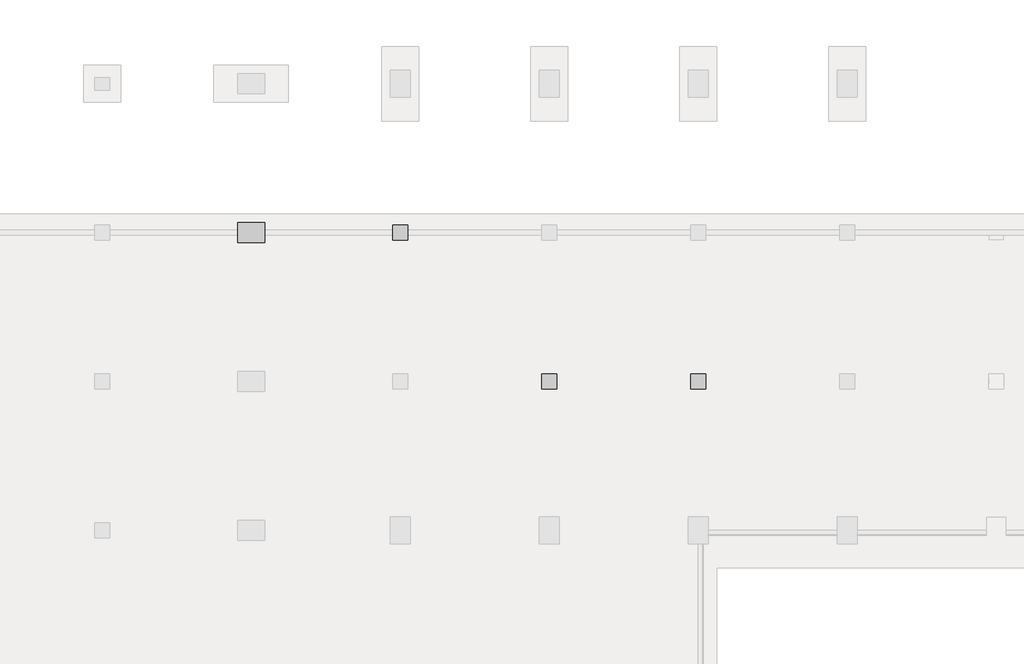
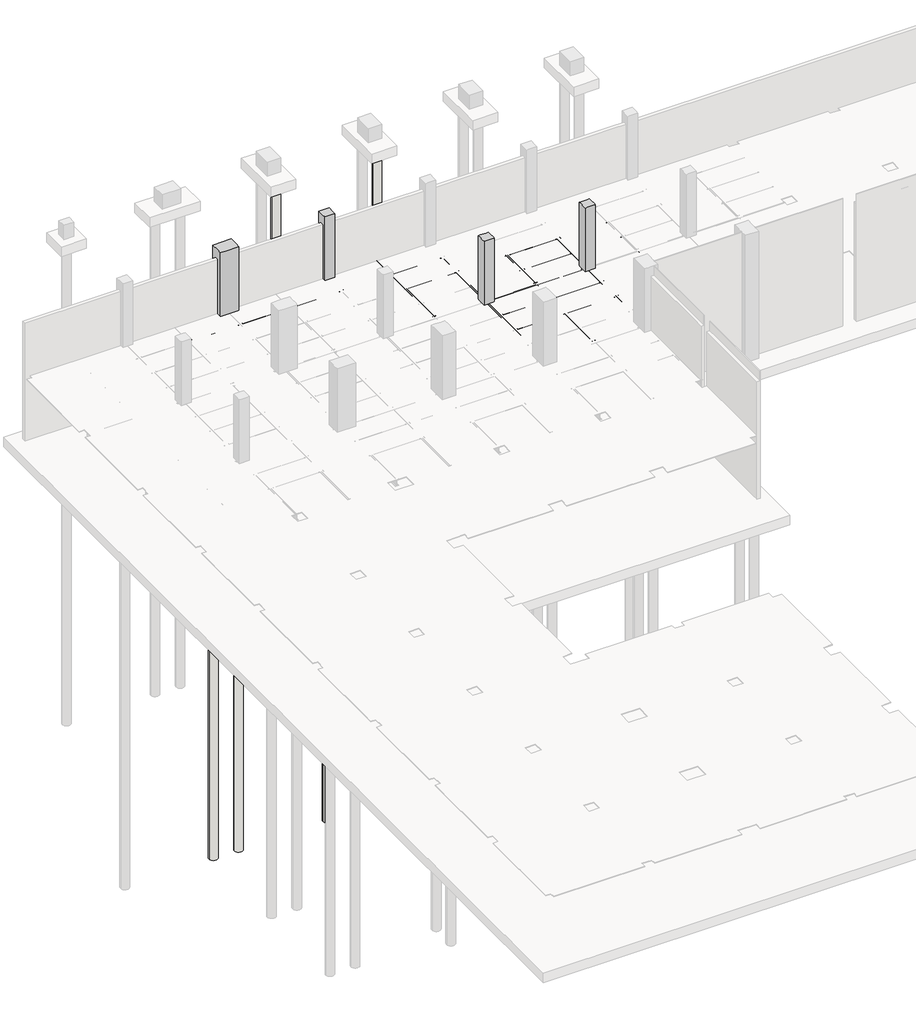
# Not in any storey, part 13 of 16: 29 beams, 6 slabs, 4 columns.
"""IFC4 building model written with IfcOpenShell, lengths in millimetres."""

from ifc_helpers import new_model, si_unit, point, frame, frame_2d, origin, place, context, project, spatial, polyline, circle_curve, trimmed, segment, composite_curve, outline, extrude, faceted_brep, element, save

model = new_model("IFC4")

# Units and contexts
model_context = context("Model", 3, world=origin())
ifc_project = project(units=[si_unit("LENGTHUNIT", "METRE", prefix="MILLI")], contexts=[model_context])

# Site, building
site = spatial("IfcSite", under=ifc_project)
building = spatial("IfcBuilding", under=site)

# Beams
placement = place(None, origin())
element("IfcBeam", 1, ObjectType="Steel Framing_C_KS : H_SB_AR_S02_C-150x75x6.5x10_J1", at=placement, inside=building, context=model_context, shape_type="SweptSolid", body=[
    extrude(outline(composite_curve([segment(polyline([(-7477.2, -3800.0381366), (-7477.2, -3950.0381366), (-7552.2, -3950.0381366)]), True, "CONTINUOUS"), segment(trimmed(circle_curve(frame_2d((-7542.2, -3950.0381366)), 10.0), [point((-7552.2, -3950.0381366))], [point((-7542.2, -3940.0381366))], False, "CARTESIAN"), True, "CONTINUOUS"), segment(polyline([(-7542.2, -3940.0381366), (-7483.7, -3930.7726469), (-7483.7, -3819.3036264), (-7542.2, -3810.0381366)]), True, "CONTINUOUS"), segment(trimmed(circle_curve(frame_2d((-7542.2, -3800.0381366)), 10.0), [point((-7542.2, -3810.0381366))], [point((-7552.2, -3800.0381366))], False, "CARTESIAN"), True, "CONTINUOUS"), segment(polyline([(-7552.2, -3800.0381366), (-7477.2, -3800.0381366)]), True, "CONTINUOUS")], self_intersect=False)), frame((33112.7, 0.0, 0.0), z_axis=(1.0, 0.0, 0.0), x_axis=(0.0, 1.0, 0.0)), (0.0, 0.0, 1.0), 2774.6),
])
element("IfcBeam", 2, ObjectType="Steel Framing_C_KS : H_SB_AR_S02_C-150x75x6.5x10_J1", at=placement, inside=building, context=model_context, shape_type="SweptSolid", body=[
    extrude(outline(composite_curve([segment(polyline([(-7477.2, -3800.0381366), (-7477.2, -3950.0381366), (-7552.2, -3950.0381366)]), True, "CONTINUOUS"), segment(trimmed(circle_curve(frame_2d((-7542.2, -3950.0381366)), 10.0), [point((-7552.2, -3950.0381366))], [point((-7542.2, -3940.0381366))], False, "CARTESIAN"), True, "CONTINUOUS"), segment(polyline([(-7542.2, -3940.0381366), (-7483.7, -3930.7726469), (-7483.7, -3819.3036264), (-7542.2, -3810.0381366)]), True, "CONTINUOUS"), segment(trimmed(circle_curve(frame_2d((-7542.2, -3800.0381366)), 10.0), [point((-7542.2, -3810.0381366))], [point((-7552.2, -3800.0381366))], False, "CARTESIAN"), True, "CONTINUOUS"), segment(polyline([(-7552.2, -3800.0381366), (-7477.2, -3800.0381366)]), True, "CONTINUOUS")], self_intersect=False)), frame((36112.7, 0.0, 0.0), z_axis=(1.0, 0.0, 0.0), x_axis=(0.0, 1.0, 0.0)), (0.0, 0.0, 1.0), 2774.6),
])
element("IfcBeam", 3, ObjectType="Steel Framing_C_KS : H_SB_AR_S02_C-150x75x6.5x10_J1", at=placement, inside=building, context=model_context, shape_type="SweptSolid", body=[
    extrude(outline(composite_curve([segment(polyline([(-7477.2, -3800.0381366), (-7477.2, -3950.0381366), (-7552.2, -3950.0381366)]), True, "CONTINUOUS"), segment(trimmed(circle_curve(frame_2d((-7542.2, -3950.0381366)), 10.0), [point((-7552.2, -3950.0381366))], [point((-7542.2, -3940.0381366))], False, "CARTESIAN"), True, "CONTINUOUS"), segment(polyline([(-7542.2, -3940.0381366), (-7483.7, -3930.7726469), (-7483.7, -3819.3036264), (-7542.2, -3810.0381366)]), True, "CONTINUOUS"), segment(trimmed(circle_curve(frame_2d((-7542.2, -3800.0381366)), 10.0), [point((-7542.2, -3810.0381366))], [point((-7552.2, -3800.0381366))], False, "CARTESIAN"), True, "CONTINUOUS"), segment(polyline([(-7552.2, -3800.0381366), (-7477.2, -3800.0381366)]), True, "CONTINUOUS")], self_intersect=False)), frame((39112.7, 0.0, 0.0), z_axis=(1.0, 0.0, 0.0), x_axis=(0.0, 1.0, 0.0)), (0.0, 0.0, 1.0), 2774.6),
])
element("IfcBeam", 4, ObjectType="Steel Framing_H_KS : H_SB_AR_S02_H-400x200x8x13_BSG2", at=placement, inside=building, context=model_context, shape_type="SweptSolid", body=[
    extrude(outline(composite_curve([segment(polyline([(-4187.0381366, 47900.0), (-4200.0381366, 47900.0), (-4200.0381366, 48100.0), (-4187.0381366, 48100.0), (-4187.0381366, 48020.0)]), True, "CONTINUOUS"), segment(trimmed(circle_curve(frame_2d((-4171.0381366, 48020.0)), 16.0), [point((-4187.0381366, 48020.0))], [point((-4171.0381366, 48004.0))], True, "CARTESIAN"), True, "CONTINUOUS"), segment(polyline([(-4171.0381366, 48004.0), (-3829.0381366, 48004.0)]), True, "CONTINUOUS"), segment(trimmed(circle_curve(frame_2d((-3829.0381366, 48020.0)), 16.0), [point((-3829.0381366, 48004.0))], [point((-3813.0381366, 48020.0))], True, "CARTESIAN"), True, "CONTINUOUS"), segment(polyline([(-3813.0381366, 48020.0), (-3813.0381366, 48100.0), (-3800.0381366, 48100.0), (-3800.0381366, 47900.0), (-3813.0381366, 47900.0), (-3813.0381366, 47980.0)]), True, "CONTINUOUS"), segment(trimmed(circle_curve(frame_2d((-3829.0381366, 47980.0)), 16.0), [point((-3813.0381366, 47980.0))], [point((-3829.0381366, 47996.0))], True, "CARTESIAN"), True, "CONTINUOUS"), segment(polyline([(-3829.0381366, 47996.0), (-4171.0381366, 47996.0)]), True, "CONTINUOUS"), segment(trimmed(circle_curve(frame_2d((-4171.0381366, 47980.0)), 16.0), [point((-4171.0381366, 47996.0))], [point((-4187.0381366, 47980.0))], True, "CARTESIAN"), True, "CONTINUOUS"), segment(polyline([(-4187.0381366, 47980.0), (-4187.0381366, 47900.0)]), True, "CONTINUOUS")], self_intersect=False)), frame((0.0, -11687.3, 0.0), z_axis=(0.0, 1.0, 0.0), x_axis=(0.0, 0.0, 1.0)), (0.0, 0.0, 1.0), 5374.6),
])
element("IfcBeam", 5, ObjectType="Steel Framing_H_KS : H_SB_AR_S02_H-400x200x8x13_BSB1", at=placement, inside=building, context=model_context, shape_type="SweptSolid", body=[
    extrude(outline(composite_curve([segment(polyline([(-4187.0381366, 44900.0), (-4200.0381366, 44900.0), (-4200.0381366, 45100.0), (-4187.0381366, 45100.0), (-4187.0381366, 45020.0)]), True, "CONTINUOUS"), segment(trimmed(circle_curve(frame_2d((-4171.0381366, 45020.0)), 16.0), [point((-4187.0381366, 45020.0))], [point((-4171.0381366, 45004.0))], True, "CARTESIAN"), True, "CONTINUOUS"), segment(polyline([(-4171.0381366, 45004.0), (-3829.0381366, 45004.0)]), True, "CONTINUOUS"), segment(trimmed(circle_curve(frame_2d((-3829.0381366, 45020.0)), 16.0), [point((-3829.0381366, 45004.0))], [point((-3813.0381366, 45020.0))], True, "CARTESIAN"), True, "CONTINUOUS"), segment(polyline([(-3813.0381366, 45020.0), (-3813.0381366, 45100.0), (-3800.0381366, 45100.0), (-3800.0381366, 44900.0), (-3813.0381366, 44900.0), (-3813.0381366, 44980.0)]), True, "CONTINUOUS"), segment(trimmed(circle_curve(frame_2d((-3829.0381366, 44980.0)), 16.0), [point((-3813.0381366, 44980.0))], [point((-3829.0381366, 44996.0))], True, "CARTESIAN"), True, "CONTINUOUS"), segment(polyline([(-3829.0381366, 44996.0), (-4171.0381366, 44996.0)]), True, "CONTINUOUS"), segment(trimmed(circle_curve(frame_2d((-4171.0381366, 44980.0)), 16.0), [point((-4171.0381366, 44996.0))], [point((-4187.0381366, 44980.0))], True, "CARTESIAN"), True, "CONTINUOUS"), segment(polyline([(-4187.0381366, 44980.0), (-4187.0381366, 44900.0)]), True, "CONTINUOUS")], self_intersect=False)), frame((0.0, -11887.3, 0.0), z_axis=(0.0, 1.0, 0.0), x_axis=(0.0, 0.0, 1.0)), (0.0, 0.0, 1.0), 5887.3),
])
element("IfcBeam", 6, ObjectType="Steel Framing_C_KS : H_SB_AR_S02_C-150x75x6.5x10_J1", at=placement, inside=building, context=model_context, shape_type="SweptSolid", body=[
    extrude(outline(composite_curve([segment(polyline([(-7477.2, -3800.0381366), (-7477.2, -3950.0381366), (-7552.2, -3950.0381366)]), True, "CONTINUOUS"), segment(trimmed(circle_curve(frame_2d((-7542.2, -3950.0381366)), 10.0), [point((-7552.2, -3950.0381366))], [point((-7542.2, -3940.0381366))], False, "CARTESIAN"), True, "CONTINUOUS"), segment(polyline([(-7542.2, -3940.0381366), (-7483.7, -3930.7726469), (-7483.7, -3819.3036264), (-7542.2, -3810.0381366)]), True, "CONTINUOUS"), segment(trimmed(circle_curve(frame_2d((-7542.2, -3800.0381366)), 10.0), [point((-7542.2, -3810.0381366))], [point((-7552.2, -3800.0381366))], False, "CARTESIAN"), True, "CONTINUOUS"), segment(polyline([(-7552.2, -3800.0381366), (-7477.2, -3800.0381366)]), True, "CONTINUOUS")], self_intersect=False)), frame((42112.7, 0.0, 0.0), z_axis=(1.0, 0.0, 0.0), x_axis=(0.0, 1.0, 0.0)), (0.0, 0.0, 1.0), 2774.6),
])
element("IfcBeam", 7, ObjectType="Steel Framing_C_KS : H_SB_AR_S02_C-150x75x6.5x10_J1", at=placement, inside=building, context=model_context, shape_type="SweptSolid", body=[
    extrude(outline(composite_curve([segment(polyline([(-8977.2, -3800.0381366), (-8977.2, -3950.0381366), (-9052.2, -3950.0381366)]), True, "CONTINUOUS"), segment(trimmed(circle_curve(frame_2d((-9042.2, -3950.0381366)), 10.0), [point((-9052.2, -3950.0381366))], [point((-9042.2, -3940.0381366))], False, "CARTESIAN"), True, "CONTINUOUS"), segment(polyline([(-9042.2, -3940.0381366), (-8983.7, -3930.7726469), (-8983.7, -3819.3036264), (-9042.2, -3810.0381366)]), True, "CONTINUOUS"), segment(trimmed(circle_curve(frame_2d((-9042.2, -3800.0381366)), 10.0), [point((-9042.2, -3810.0381366))], [point((-9052.2, -3800.0381366))], False, "CARTESIAN"), True, "CONTINUOUS"), segment(polyline([(-9052.2, -3800.0381366), (-8977.2, -3800.0381366)]), True, "CONTINUOUS")], self_intersect=False)), frame((45112.7, 0.0, 0.0), z_axis=(1.0, 0.0, 0.0), x_axis=(0.0, 1.0, 0.0)), (0.0, 0.0, 1.0), 2774.6),
])
element("IfcBeam", 8, ObjectType="Steel Framing_C_KS : H_SB_AR_S02_C-150x75x6.5x10_J1", at=placement, inside=building, context=model_context, shape_type="SweptSolid", body=[
    extrude(outline(composite_curve([segment(polyline([(-7477.2, -3800.0381366), (-7477.2, -3950.0381366), (-7552.2, -3950.0381366)]), True, "CONTINUOUS"), segment(trimmed(circle_curve(frame_2d((-7542.2, -3950.0381366)), 10.0), [point((-7552.2, -3950.0381366))], [point((-7542.2, -3940.0381366))], False, "CARTESIAN"), True, "CONTINUOUS"), segment(polyline([(-7542.2, -3940.0381366), (-7483.7, -3930.7726469), (-7483.7, -3819.3036264), (-7542.2, -3810.0381366)]), True, "CONTINUOUS"), segment(trimmed(circle_curve(frame_2d((-7542.2, -3800.0381366)), 10.0), [point((-7542.2, -3810.0381366))], [point((-7552.2, -3800.0381366))], False, "CARTESIAN"), True, "CONTINUOUS"), segment(polyline([(-7552.2, -3800.0381366), (-7477.2, -3800.0381366)]), True, "CONTINUOUS")], self_intersect=False)), frame((45112.7, 0.0, 0.0), z_axis=(1.0, 0.0, 0.0), x_axis=(0.0, 1.0, 0.0)), (0.0, 0.0, 1.0), 2774.6),
])
element("IfcBeam", 9, ObjectType="Steel Framing_H_KS : H_SB_AR_S02_H-400x200x8x13_BSG1", at=placement, inside=building, context=model_context, shape_type="SweptSolid", body=[
    extrude(outline(composite_curve([segment(polyline([(-11900.0, -4187.0381366), (-11900.0, -4200.0381366), (-12100.0, -4200.0381366), (-12100.0, -4187.0381366), (-12020.0, -4187.0381366)]), True, "CONTINUOUS"), segment(trimmed(circle_curve(frame_2d((-12020.0, -4171.0381366)), 16.0), [point((-12020.0, -4187.0381366))], [point((-12004.0, -4171.0381366))], True, "CARTESIAN"), True, "CONTINUOUS"), segment(polyline([(-12004.0, -4171.0381366), (-12004.0, -3829.0381366)]), True, "CONTINUOUS"), segment(trimmed(circle_curve(frame_2d((-12020.0, -3829.0381366)), 16.0), [point((-12004.0, -3829.0381366))], [point((-12020.0, -3813.0381366))], True, "CARTESIAN"), True, "CONTINUOUS"), segment(polyline([(-12020.0, -3813.0381366), (-12100.0, -3813.0381366), (-12100.0, -3800.0381366), (-11900.0, -3800.0381366), (-11900.0, -3813.0381366), (-11980.0, -3813.0381366)]), True, "CONTINUOUS"), segment(trimmed(circle_curve(frame_2d((-11980.0, -3829.0381366)), 16.0), [point((-11980.0, -3813.0381366))], [point((-11996.0, -3829.0381366))], True, "CARTESIAN"), True, "CONTINUOUS"), segment(polyline([(-11996.0, -3829.0381366), (-11996.0, -4171.0381366)]), True, "CONTINUOUS"), segment(trimmed(circle_curve(frame_2d((-11980.0, -4171.0381366)), 16.0), [point((-11996.0, -4171.0381366))], [point((-11980.0, -4187.0381366))], True, "CARTESIAN"), True, "CONTINUOUS"), segment(polyline([(-11980.0, -4187.0381366), (-11900.0, -4187.0381366)]), True, "CONTINUOUS")], self_intersect=False)), frame((48312.7, 0.0, 0.0), z_axis=(1.0, 0.0, 0.0), x_axis=(0.0, 1.0, 0.0)), (0.0, 0.0, 1.0), 5374.6),
])
element("IfcBeam", 10, ObjectType="Steel Framing_H_KS : H_SB_AR_S02_H-400x200x8x13_BSG2", at=placement, inside=building, context=model_context, shape_type="SweptSolid", body=[
    extrude(outline(composite_curve([segment(polyline([(-4187.0381366, 53900.0), (-4200.0381366, 53900.0), (-4200.0381366, 54100.0), (-4187.0381366, 54100.0), (-4187.0381366, 54020.0)]), True, "CONTINUOUS"), segment(trimmed(circle_curve(frame_2d((-4171.0381366, 54020.0)), 16.0), [point((-4187.0381366, 54020.0))], [point((-4171.0381366, 54004.0))], True, "CARTESIAN"), True, "CONTINUOUS"), segment(polyline([(-4171.0381366, 54004.0), (-3829.0381366, 54004.0)]), True, "CONTINUOUS"), segment(trimmed(circle_curve(frame_2d((-3829.0381366, 54020.0)), 16.0), [point((-3829.0381366, 54004.0))], [point((-3813.0381366, 54020.0))], True, "CARTESIAN"), True, "CONTINUOUS"), segment(polyline([(-3813.0381366, 54020.0), (-3813.0381366, 54100.0), (-3800.0381366, 54100.0), (-3800.0381366, 53900.0), (-3813.0381366, 53900.0), (-3813.0381366, 53980.0)]), True, "CONTINUOUS"), segment(trimmed(circle_curve(frame_2d((-3829.0381366, 53980.0)), 16.0), [point((-3813.0381366, 53980.0))], [point((-3829.0381366, 53996.0))], True, "CARTESIAN"), True, "CONTINUOUS"), segment(polyline([(-3829.0381366, 53996.0), (-4171.0381366, 53996.0)]), True, "CONTINUOUS"), segment(trimmed(circle_curve(frame_2d((-4171.0381366, 53980.0)), 16.0), [point((-4171.0381366, 53996.0))], [point((-4187.0381366, 53980.0))], True, "CARTESIAN"), True, "CONTINUOUS"), segment(polyline([(-4187.0381366, 53980.0), (-4187.0381366, 53900.0)]), True, "CONTINUOUS")], self_intersect=False)), frame((0.0, -11687.3, 0.0), z_axis=(0.0, 1.0, 0.0), x_axis=(0.0, 0.0, 1.0)), (0.0, 0.0, 1.0), 5374.6),
])
element("IfcBeam", 11, ObjectType="Steel Framing_H_KS : H_SB_AR_S02_H-400x200x8x13_BSB1", at=placement, inside=building, context=model_context, shape_type="SweptSolid", body=[
    extrude(outline(composite_curve([segment(polyline([(-4187.0381366, 50900.0), (-4200.0381366, 50900.0), (-4200.0381366, 51100.0), (-4187.0381366, 51100.0), (-4187.0381366, 51020.0)]), True, "CONTINUOUS"), segment(trimmed(circle_curve(frame_2d((-4171.0381366, 51020.0)), 16.0), [point((-4187.0381366, 51020.0))], [point((-4171.0381366, 51004.0))], True, "CARTESIAN"), True, "CONTINUOUS"), segment(polyline([(-4171.0381366, 51004.0), (-3829.0381366, 51004.0)]), True, "CONTINUOUS"), segment(trimmed(circle_curve(frame_2d((-3829.0381366, 51020.0)), 16.0), [point((-3829.0381366, 51004.0))], [point((-3813.0381366, 51020.0))], True, "CARTESIAN"), True, "CONTINUOUS"), segment(polyline([(-3813.0381366, 51020.0), (-3813.0381366, 51100.0), (-3800.0381366, 51100.0), (-3800.0381366, 50900.0), (-3813.0381366, 50900.0), (-3813.0381366, 50980.0)]), True, "CONTINUOUS"), segment(trimmed(circle_curve(frame_2d((-3829.0381366, 50980.0)), 16.0), [point((-3813.0381366, 50980.0))], [point((-3829.0381366, 50996.0))], True, "CARTESIAN"), True, "CONTINUOUS"), segment(polyline([(-3829.0381366, 50996.0), (-4171.0381366, 50996.0)]), True, "CONTINUOUS"), segment(trimmed(circle_curve(frame_2d((-4171.0381366, 50980.0)), 16.0), [point((-4171.0381366, 50996.0))], [point((-4187.0381366, 50980.0))], True, "CARTESIAN"), True, "CONTINUOUS"), segment(polyline([(-4187.0381366, 50980.0), (-4187.0381366, 50900.0)]), True, "CONTINUOUS")], self_intersect=False)), frame((0.0, -11887.3, 0.0), z_axis=(0.0, 1.0, 0.0), x_axis=(0.0, 0.0, 1.0)), (0.0, 0.0, 1.0), 5887.3),
])
element("IfcBeam", 12, ObjectType="Steel Framing_C_KS : H_SB_AR_S02_C-150x75x6.5x10_J1", at=placement, inside=building, context=model_context, shape_type="SweptSolid", body=[
    extrude(outline(composite_curve([segment(polyline([(-8977.2, -3800.0381366), (-8977.2, -3950.0381366), (-9052.2, -3950.0381366)]), True, "CONTINUOUS"), segment(trimmed(circle_curve(frame_2d((-9042.2, -3950.0381366)), 10.0), [point((-9052.2, -3950.0381366))], [point((-9042.2, -3940.0381366))], False, "CARTESIAN"), True, "CONTINUOUS"), segment(polyline([(-9042.2, -3940.0381366), (-8983.7, -3930.7726469), (-8983.7, -3819.3036264), (-9042.2, -3810.0381366)]), True, "CONTINUOUS"), segment(trimmed(circle_curve(frame_2d((-9042.2, -3800.0381366)), 10.0), [point((-9042.2, -3810.0381366))], [point((-9052.2, -3800.0381366))], False, "CARTESIAN"), True, "CONTINUOUS"), segment(polyline([(-9052.2, -3800.0381366), (-8977.2, -3800.0381366)]), True, "CONTINUOUS")], self_intersect=False)), frame((48112.7, 0.0, 0.0), z_axis=(1.0, 0.0, 0.0), x_axis=(0.0, 1.0, 0.0)), (0.0, 0.0, 1.0), 2774.6),
])
element("IfcBeam", 13, ObjectType="Steel Framing_C_KS : H_SB_AR_S02_C-150x75x6.5x10_J1", at=placement, inside=building, context=model_context, shape_type="SweptSolid", body=[
    extrude(outline(composite_curve([segment(polyline([(-10477.2, -3800.0381366), (-10477.2, -3950.0381366), (-10552.2, -3950.0381366)]), True, "CONTINUOUS"), segment(trimmed(circle_curve(frame_2d((-10542.2, -3950.0381366)), 10.0), [point((-10552.2, -3950.0381366))], [point((-10542.2, -3940.0381366))], False, "CARTESIAN"), True, "CONTINUOUS"), segment(polyline([(-10542.2, -3940.0381366), (-10483.7, -3930.7726469), (-10483.7, -3819.3036264), (-10542.2, -3810.0381366)]), True, "CONTINUOUS"), segment(trimmed(circle_curve(frame_2d((-10542.2, -3800.0381366)), 10.0), [point((-10542.2, -3810.0381366))], [point((-10552.2, -3800.0381366))], False, "CARTESIAN"), True, "CONTINUOUS"), segment(polyline([(-10552.2, -3800.0381366), (-10477.2, -3800.0381366)]), True, "CONTINUOUS")], self_intersect=False)), frame((48112.7, 0.0, 0.0), z_axis=(1.0, 0.0, 0.0), x_axis=(0.0, 1.0, 0.0)), (0.0, 0.0, 1.0), 2774.6),
])
element("IfcBeam", 14, ObjectType="Steel Framing_C_KS : H_SB_AR_S02_C-150x75x6.5x10_J1", at=placement, inside=building, context=model_context, shape_type="SweptSolid", body=[
    extrude(outline(composite_curve([segment(polyline([(-8977.2, -3800.0381366), (-8977.2, -3950.0381366), (-9052.2, -3950.0381366)]), True, "CONTINUOUS"), segment(trimmed(circle_curve(frame_2d((-9042.2, -3950.0381366)), 10.0), [point((-9052.2, -3950.0381366))], [point((-9042.2, -3940.0381366))], False, "CARTESIAN"), True, "CONTINUOUS"), segment(polyline([(-9042.2, -3940.0381366), (-8983.7, -3930.7726469), (-8983.7, -3819.3036264), (-9042.2, -3810.0381366)]), True, "CONTINUOUS"), segment(trimmed(circle_curve(frame_2d((-9042.2, -3800.0381366)), 10.0), [point((-9042.2, -3810.0381366))], [point((-9052.2, -3800.0381366))], False, "CARTESIAN"), True, "CONTINUOUS"), segment(polyline([(-9052.2, -3800.0381366), (-8977.2, -3800.0381366)]), True, "CONTINUOUS")], self_intersect=False)), frame((51112.7, 0.0, 0.0), z_axis=(1.0, 0.0, 0.0), x_axis=(0.0, 1.0, 0.0)), (0.0, 0.0, 1.0), 2774.6),
])
element("IfcBeam", 15, ObjectType="Steel Framing_C_KS : H_SB_AR_S02_C-150x75x6.5x10_J1", at=placement, inside=building, context=model_context, shape_type="SweptSolid", body=[
    extrude(outline(composite_curve([segment(polyline([(-10477.2, -3800.0381366), (-10477.2, -3950.0381366), (-10552.2, -3950.0381366)]), True, "CONTINUOUS"), segment(trimmed(circle_curve(frame_2d((-10542.2, -3950.0381366)), 10.0), [point((-10552.2, -3950.0381366))], [point((-10542.2, -3940.0381366))], False, "CARTESIAN"), True, "CONTINUOUS"), segment(polyline([(-10542.2, -3940.0381366), (-10483.7, -3930.7726469), (-10483.7, -3819.3036264), (-10542.2, -3810.0381366)]), True, "CONTINUOUS"), segment(trimmed(circle_curve(frame_2d((-10542.2, -3800.0381366)), 10.0), [point((-10542.2, -3810.0381366))], [point((-10552.2, -3800.0381366))], False, "CARTESIAN"), True, "CONTINUOUS"), segment(polyline([(-10552.2, -3800.0381366), (-10477.2, -3800.0381366)]), True, "CONTINUOUS")], self_intersect=False)), frame((51112.7, 0.0, 0.0), z_axis=(1.0, 0.0, 0.0), x_axis=(0.0, 1.0, 0.0)), (0.0, 0.0, 1.0), 2774.6),
])
element("IfcBeam", 16, ObjectType="Steel Framing_C_KS : H_SB_AR_S02_C-150x75x6.5x10_J1", at=placement, inside=building, context=model_context, shape_type="SweptSolid", body=[
    extrude(outline(composite_curve([segment(polyline([(-8977.2, -3800.0381366), (-8977.2, -3950.0381366), (-9052.2, -3950.0381366)]), True, "CONTINUOUS"), segment(trimmed(circle_curve(frame_2d((-9042.2, -3950.0381366)), 10.0), [point((-9052.2, -3950.0381366))], [point((-9042.2, -3940.0381366))], False, "CARTESIAN"), True, "CONTINUOUS"), segment(polyline([(-9042.2, -3940.0381366), (-8983.7, -3930.7726469), (-8983.7, -3819.3036264), (-9042.2, -3810.0381366)]), True, "CONTINUOUS"), segment(trimmed(circle_curve(frame_2d((-9042.2, -3800.0381366)), 10.0), [point((-9042.2, -3810.0381366))], [point((-9052.2, -3800.0381366))], False, "CARTESIAN"), True, "CONTINUOUS"), segment(polyline([(-9052.2, -3800.0381366), (-8977.2, -3800.0381366)]), True, "CONTINUOUS")], self_intersect=False)), frame((54112.7, 0.0, 0.0), z_axis=(1.0, 0.0, 0.0), x_axis=(0.0, 1.0, 0.0)), (0.0, 0.0, 1.0), 2774.6),
])
element("IfcBeam", 17, ObjectType="Steel Framing_C_KS : H_SB_AR_S02_C-150x75x6.5x10_J1", at=placement, inside=building, context=model_context, shape_type="SweptSolid", body=[
    extrude(outline(composite_curve([segment(polyline([(-10477.2, -3800.0381366), (-10477.2, -3950.0381366), (-10552.2, -3950.0381366)]), True, "CONTINUOUS"), segment(trimmed(circle_curve(frame_2d((-10542.2, -3950.0381366)), 10.0), [point((-10552.2, -3950.0381366))], [point((-10542.2, -3940.0381366))], False, "CARTESIAN"), True, "CONTINUOUS"), segment(polyline([(-10542.2, -3940.0381366), (-10483.7, -3930.7726469), (-10483.7, -3819.3036264), (-10542.2, -3810.0381366)]), True, "CONTINUOUS"), segment(trimmed(circle_curve(frame_2d((-10542.2, -3800.0381366)), 10.0), [point((-10542.2, -3810.0381366))], [point((-10552.2, -3800.0381366))], False, "CARTESIAN"), True, "CONTINUOUS"), segment(polyline([(-10552.2, -3800.0381366), (-10477.2, -3800.0381366)]), True, "CONTINUOUS")], self_intersect=False)), frame((54112.7, 0.0, 0.0), z_axis=(1.0, 0.0, 0.0), x_axis=(0.0, 1.0, 0.0)), (0.0, 0.0, 1.0), 2774.6),
])
element("IfcBeam", 18, ObjectType="Steel Framing_H_KS : H_SB_AR_S02_H-400x200x8x13_BSG2", at=placement, inside=building, context=model_context, shape_type="SweptSolid", body=[
    extrude(outline(composite_curve([segment(polyline([(-4187.0381366, 47900.0), (-4200.0381366, 47900.0), (-4200.0381366, 48100.0), (-4187.0381366, 48100.0), (-4187.0381366, 48020.0)]), True, "CONTINUOUS"), segment(trimmed(circle_curve(frame_2d((-4171.0381366, 48020.0)), 16.0), [point((-4187.0381366, 48020.0))], [point((-4171.0381366, 48004.0))], True, "CARTESIAN"), True, "CONTINUOUS"), segment(polyline([(-4171.0381366, 48004.0), (-3829.0381366, 48004.0)]), True, "CONTINUOUS"), segment(trimmed(circle_curve(frame_2d((-3829.0381366, 48020.0)), 16.0), [point((-3829.0381366, 48004.0))], [point((-3813.0381366, 48020.0))], True, "CARTESIAN"), True, "CONTINUOUS"), segment(polyline([(-3813.0381366, 48020.0), (-3813.0381366, 48100.0), (-3800.0381366, 48100.0), (-3800.0381366, 47900.0), (-3813.0381366, 47900.0), (-3813.0381366, 47980.0)]), True, "CONTINUOUS"), segment(trimmed(circle_curve(frame_2d((-3829.0381366, 47980.0)), 16.0), [point((-3813.0381366, 47980.0))], [point((-3829.0381366, 47996.0))], True, "CARTESIAN"), True, "CONTINUOUS"), segment(polyline([(-3829.0381366, 47996.0), (-4171.0381366, 47996.0)]), True, "CONTINUOUS"), segment(trimmed(circle_curve(frame_2d((-4171.0381366, 47980.0)), 16.0), [point((-4171.0381366, 47996.0))], [point((-4187.0381366, 47980.0))], True, "CARTESIAN"), True, "CONTINUOUS"), segment(polyline([(-4187.0381366, 47980.0), (-4187.0381366, 47900.0)]), True, "CONTINUOUS")], self_intersect=False)), frame((0.0, -17437.3, 0.0), z_axis=(0.0, 1.0, 0.0), x_axis=(0.0, 0.0, 1.0)), (0.0, 0.0, 1.0), 5124.6),
])
element("IfcBeam", 19, ObjectType="Steel Framing_H_KS : H_SB_AR_S02_H-400x200x8x13_BSG2", at=placement, inside=building, context=model_context, shape_type="SweptSolid", body=[
    extrude(outline(composite_curve([segment(polyline([(-4187.0381366, 53900.0), (-4200.0381366, 53900.0), (-4200.0381366, 54100.0), (-4187.0381366, 54100.0), (-4187.0381366, 54020.0)]), True, "CONTINUOUS"), segment(trimmed(circle_curve(frame_2d((-4171.0381366, 54020.0)), 16.0), [point((-4187.0381366, 54020.0))], [point((-4171.0381366, 54004.0))], True, "CARTESIAN"), True, "CONTINUOUS"), segment(polyline([(-4171.0381366, 54004.0), (-3829.0381366, 54004.0)]), True, "CONTINUOUS"), segment(trimmed(circle_curve(frame_2d((-3829.0381366, 54020.0)), 16.0), [point((-3829.0381366, 54004.0))], [point((-3813.0381366, 54020.0))], True, "CARTESIAN"), True, "CONTINUOUS"), segment(polyline([(-3813.0381366, 54020.0), (-3813.0381366, 54100.0), (-3800.0381366, 54100.0), (-3800.0381366, 53900.0), (-3813.0381366, 53900.0), (-3813.0381366, 53980.0)]), True, "CONTINUOUS"), segment(trimmed(circle_curve(frame_2d((-3829.0381366, 53980.0)), 16.0), [point((-3813.0381366, 53980.0))], [point((-3829.0381366, 53996.0))], True, "CARTESIAN"), True, "CONTINUOUS"), segment(polyline([(-3829.0381366, 53996.0), (-4171.0381366, 53996.0)]), True, "CONTINUOUS"), segment(trimmed(circle_curve(frame_2d((-4171.0381366, 53980.0)), 16.0), [point((-4171.0381366, 53996.0))], [point((-4187.0381366, 53980.0))], True, "CARTESIAN"), True, "CONTINUOUS"), segment(polyline([(-4187.0381366, 53980.0), (-4187.0381366, 53900.0)]), True, "CONTINUOUS")], self_intersect=False)), frame((0.0, -17437.3, 0.0), z_axis=(0.0, 1.0, 0.0), x_axis=(0.0, 0.0, 1.0)), (0.0, 0.0, 1.0), 5124.6),
])
element("IfcBeam", 20, ObjectType="Steel Framing_H_KS : H_SB_AR_S02_H-400x200x8x13_BSB1", at=placement, inside=building, context=model_context, shape_type="SweptSolid", body=[
    extrude(outline(composite_curve([segment(polyline([(-4187.0381366, 50900.0), (-4200.0381366, 50900.0), (-4200.0381366, 51100.0), (-4187.0381366, 51100.0), (-4187.0381366, 51020.0)]), True, "CONTINUOUS"), segment(trimmed(circle_curve(frame_2d((-4171.0381366, 51020.0)), 16.0), [point((-4187.0381366, 51020.0))], [point((-4171.0381366, 51004.0))], True, "CARTESIAN"), True, "CONTINUOUS"), segment(polyline([(-4171.0381366, 51004.0), (-3829.0381366, 51004.0)]), True, "CONTINUOUS"), segment(trimmed(circle_curve(frame_2d((-3829.0381366, 51020.0)), 16.0), [point((-3829.0381366, 51004.0))], [point((-3813.0381366, 51020.0))], True, "CARTESIAN"), True, "CONTINUOUS"), segment(polyline([(-3813.0381366, 51020.0), (-3813.0381366, 51100.0), (-3800.0381366, 51100.0), (-3800.0381366, 50900.0), (-3813.0381366, 50900.0), (-3813.0381366, 50980.0)]), True, "CONTINUOUS"), segment(trimmed(circle_curve(frame_2d((-3829.0381366, 50980.0)), 16.0), [point((-3813.0381366, 50980.0))], [point((-3829.0381366, 50996.0))], True, "CARTESIAN"), True, "CONTINUOUS"), segment(polyline([(-3829.0381366, 50996.0), (-4171.0381366, 50996.0)]), True, "CONTINUOUS"), segment(trimmed(circle_curve(frame_2d((-4171.0381366, 50980.0)), 16.0), [point((-4171.0381366, 50996.0))], [point((-4187.0381366, 50980.0))], True, "CARTESIAN"), True, "CONTINUOUS"), segment(polyline([(-4187.0381366, 50980.0), (-4187.0381366, 50900.0)]), True, "CONTINUOUS")], self_intersect=False)), frame((0.0, -17887.3, 0.0), z_axis=(0.0, 1.0, 0.0), x_axis=(0.0, 0.0, 1.0)), (0.0, 0.0, 1.0), 5774.6),
])
element("IfcBeam", 21, ObjectType="Steel Framing_C_KS : H_SB_AR_S02_C-150x75x6.5x10_J1", at=placement, inside=building, context=model_context, shape_type="SweptSolid", body=[
    extrude(outline(composite_curve([segment(polyline([(-14977.2, -3800.0381366), (-14977.2, -3950.0381366), (-15052.2, -3950.0381366)]), True, "CONTINUOUS"), segment(trimmed(circle_curve(frame_2d((-15042.2, -3950.0381366)), 10.0), [point((-15052.2, -3950.0381366))], [point((-15042.2, -3940.0381366))], False, "CARTESIAN"), True, "CONTINUOUS"), segment(polyline([(-15042.2, -3940.0381366), (-14983.7, -3930.7726469), (-14983.7, -3819.3036264), (-15042.2, -3810.0381366)]), True, "CONTINUOUS"), segment(trimmed(circle_curve(frame_2d((-15042.2, -3800.0381366)), 10.0), [point((-15042.2, -3810.0381366))], [point((-15052.2, -3800.0381366))], False, "CARTESIAN"), True, "CONTINUOUS"), segment(polyline([(-15052.2, -3800.0381366), (-14977.2, -3800.0381366)]), True, "CONTINUOUS")], self_intersect=False)), frame((48112.7, 0.0, 0.0), z_axis=(1.0, 0.0, 0.0), x_axis=(0.0, 1.0, 0.0)), (0.0, 0.0, 1.0), 2774.6),
])
element("IfcBeam", 22, ObjectType="Steel Framing_C_KS : H_SB_AR_S02_C-150x75x6.5x10_J1", at=placement, inside=building, context=model_context, shape_type="SweptSolid", body=[
    extrude(outline(composite_curve([segment(polyline([(-13477.2, -3800.0381366), (-13477.2, -3950.0381366), (-13552.2, -3950.0381366)]), True, "CONTINUOUS"), segment(trimmed(circle_curve(frame_2d((-13542.2, -3950.0381366)), 10.0), [point((-13552.2, -3950.0381366))], [point((-13542.2, -3940.0381366))], False, "CARTESIAN"), True, "CONTINUOUS"), segment(polyline([(-13542.2, -3940.0381366), (-13483.7, -3930.7726469), (-13483.7, -3819.3036264), (-13542.2, -3810.0381366)]), True, "CONTINUOUS"), segment(trimmed(circle_curve(frame_2d((-13542.2, -3800.0381366)), 10.0), [point((-13542.2, -3810.0381366))], [point((-13552.2, -3800.0381366))], False, "CARTESIAN"), True, "CONTINUOUS"), segment(polyline([(-13552.2, -3800.0381366), (-13477.2, -3800.0381366)]), True, "CONTINUOUS")], self_intersect=False)), frame((48112.7, 0.0, 0.0), z_axis=(1.0, 0.0, 0.0), x_axis=(0.0, 1.0, 0.0)), (0.0, 0.0, 1.0), 2774.6),
])
element("IfcBeam", 23, ObjectType="Steel Framing_C_KS : H_SB_AR_S02_C-150x75x6.5x10_J1", at=placement, inside=building, context=model_context, shape_type="SweptSolid", body=[
    extrude(outline(composite_curve([segment(polyline([(-14977.2, -3800.0381366), (-14977.2, -3950.0381366), (-15052.2, -3950.0381366)]), True, "CONTINUOUS"), segment(trimmed(circle_curve(frame_2d((-15042.2, -3950.0381366)), 10.0), [point((-15052.2, -3950.0381366))], [point((-15042.2, -3940.0381366))], False, "CARTESIAN"), True, "CONTINUOUS"), segment(polyline([(-15042.2, -3940.0381366), (-14983.7, -3930.7726469), (-14983.7, -3819.3036264), (-15042.2, -3810.0381366)]), True, "CONTINUOUS"), segment(trimmed(circle_curve(frame_2d((-15042.2, -3800.0381366)), 10.0), [point((-15042.2, -3810.0381366))], [point((-15052.2, -3800.0381366))], False, "CARTESIAN"), True, "CONTINUOUS"), segment(polyline([(-15052.2, -3800.0381366), (-14977.2, -3800.0381366)]), True, "CONTINUOUS")], self_intersect=False)), frame((51112.7, 0.0, 0.0), z_axis=(1.0, 0.0, 0.0), x_axis=(0.0, 1.0, 0.0)), (0.0, 0.0, 1.0), 2774.6),
])
element("IfcBeam", 24, ObjectType="Steel Framing_C_KS : H_SB_AR_S02_C-150x75x6.5x10_J1", at=placement, inside=building, context=model_context, shape_type="SweptSolid", body=[
    extrude(outline(composite_curve([segment(polyline([(-13477.2, -3800.0381366), (-13477.2, -3950.0381366), (-13552.2, -3950.0381366)]), True, "CONTINUOUS"), segment(trimmed(circle_curve(frame_2d((-13542.2, -3950.0381366)), 10.0), [point((-13552.2, -3950.0381366))], [point((-13542.2, -3940.0381366))], False, "CARTESIAN"), True, "CONTINUOUS"), segment(polyline([(-13542.2, -3940.0381366), (-13483.7, -3930.7726469), (-13483.7, -3819.3036264), (-13542.2, -3810.0381366)]), True, "CONTINUOUS"), segment(trimmed(circle_curve(frame_2d((-13542.2, -3800.0381366)), 10.0), [point((-13542.2, -3810.0381366))], [point((-13552.2, -3800.0381366))], False, "CARTESIAN"), True, "CONTINUOUS"), segment(polyline([(-13552.2, -3800.0381366), (-13477.2, -3800.0381366)]), True, "CONTINUOUS")], self_intersect=False)), frame((51112.7, 0.0, 0.0), z_axis=(1.0, 0.0, 0.0), x_axis=(0.0, 1.0, 0.0)), (0.0, 0.0, 1.0), 2774.6),
])
element("IfcBeam", 25, ObjectType="Steel Framing_H_KS : H_SB_AR_S02_H-400x200x8x13_BSB1", at=placement, inside=building, context=model_context, shape_type="SweptSolid", body=[
    extrude(outline(composite_curve([segment(polyline([(-4187.0381366, 56900.0), (-4200.0381366, 56900.0), (-4200.0381366, 57100.0), (-4187.0381366, 57100.0), (-4187.0381366, 57020.0)]), True, "CONTINUOUS"), segment(trimmed(circle_curve(frame_2d((-4171.0381366, 57020.0)), 16.0), [point((-4187.0381366, 57020.0))], [point((-4171.0381366, 57004.0))], True, "CARTESIAN"), True, "CONTINUOUS"), segment(polyline([(-4171.0381366, 57004.0), (-3829.0381366, 57004.0)]), True, "CONTINUOUS"), segment(trimmed(circle_curve(frame_2d((-3829.0381366, 57020.0)), 16.0), [point((-3829.0381366, 57004.0))], [point((-3813.0381366, 57020.0))], True, "CARTESIAN"), True, "CONTINUOUS"), segment(polyline([(-3813.0381366, 57020.0), (-3813.0381366, 57100.0), (-3800.0381366, 57100.0), (-3800.0381366, 56900.0), (-3813.0381366, 56900.0), (-3813.0381366, 56980.0)]), True, "CONTINUOUS"), segment(trimmed(circle_curve(frame_2d((-3829.0381366, 56980.0)), 16.0), [point((-3813.0381366, 56980.0))], [point((-3829.0381366, 56996.0))], True, "CARTESIAN"), True, "CONTINUOUS"), segment(polyline([(-3829.0381366, 56996.0), (-4171.0381366, 56996.0)]), True, "CONTINUOUS"), segment(trimmed(circle_curve(frame_2d((-4171.0381366, 56980.0)), 16.0), [point((-4171.0381366, 56996.0))], [point((-4187.0381366, 56980.0))], True, "CARTESIAN"), True, "CONTINUOUS"), segment(polyline([(-4187.0381366, 56980.0), (-4187.0381366, 56900.0)]), True, "CONTINUOUS")], self_intersect=False)), frame((0.0, -18000.0, 0.0), z_axis=(0.0, 1.0, 0.0), x_axis=(0.0, 0.0, 1.0)), (0.0, 0.0, 1.0), 5887.3),
])
element("IfcBeam", 26, ObjectType="Steel Framing_C_KS : H_SB_AR_S02_C-150x75x6.5x10_J1", at=placement, inside=building, context=model_context, shape_type="SweptSolid", body=[
    extrude(outline(composite_curve([segment(polyline([(-14977.2, -3800.0381366), (-14977.2, -3950.0381366), (-15052.2, -3950.0381366)]), True, "CONTINUOUS"), segment(trimmed(circle_curve(frame_2d((-15042.2, -3950.0381366)), 10.0), [point((-15052.2, -3950.0381366))], [point((-15042.2, -3940.0381366))], False, "CARTESIAN"), True, "CONTINUOUS"), segment(polyline([(-15042.2, -3940.0381366), (-14983.7, -3930.7726469), (-14983.7, -3819.3036264), (-15042.2, -3810.0381366)]), True, "CONTINUOUS"), segment(trimmed(circle_curve(frame_2d((-15042.2, -3800.0381366)), 10.0), [point((-15042.2, -3810.0381366))], [point((-15052.2, -3800.0381366))], False, "CARTESIAN"), True, "CONTINUOUS"), segment(polyline([(-15052.2, -3800.0381366), (-14977.2, -3800.0381366)]), True, "CONTINUOUS")], self_intersect=False)), frame((54112.7, 0.0, 0.0), z_axis=(1.0, 0.0, 0.0), x_axis=(0.0, 1.0, 0.0)), (0.0, 0.0, 1.0), 2774.6),
])
element("IfcBeam", 27, ObjectType="Steel Framing_C_KS : H_SB_AR_S02_C-150x75x6.5x10_J1", at=placement, inside=building, context=model_context, shape_type="SweptSolid", body=[
    extrude(outline(composite_curve([segment(polyline([(-13477.2, -3800.0381366), (-13477.2, -3950.0381366), (-13552.2, -3950.0381366)]), True, "CONTINUOUS"), segment(trimmed(circle_curve(frame_2d((-13542.2, -3950.0381366)), 10.0), [point((-13552.2, -3950.0381366))], [point((-13542.2, -3940.0381366))], False, "CARTESIAN"), True, "CONTINUOUS"), segment(polyline([(-13542.2, -3940.0381366), (-13483.7, -3930.7726469), (-13483.7, -3819.3036264), (-13542.2, -3810.0381366)]), True, "CONTINUOUS"), segment(trimmed(circle_curve(frame_2d((-13542.2, -3800.0381366)), 10.0), [point((-13542.2, -3810.0381366))], [point((-13552.2, -3800.0381366))], False, "CARTESIAN"), True, "CONTINUOUS"), segment(polyline([(-13552.2, -3800.0381366), (-13477.2, -3800.0381366)]), True, "CONTINUOUS")], self_intersect=False)), frame((54112.7, 0.0, 0.0), z_axis=(1.0, 0.0, 0.0), x_axis=(0.0, 1.0, 0.0)), (0.0, 0.0, 1.0), 2774.6),
])
element("IfcBeam", 28, ObjectType="Steel Framing_C_KS : H_SB_AR_S02_C-150x75x6.5x10_J1", at=placement, inside=building, context=model_context, shape_type="SweptSolid", body=[
    extrude(outline(composite_curve([segment(polyline([(-14977.2, -3800.0381366), (-14977.2, -3950.0381366), (-15052.2, -3950.0381366)]), True, "CONTINUOUS"), segment(trimmed(circle_curve(frame_2d((-15042.2, -3950.0381366)), 10.0), [point((-15052.2, -3950.0381366))], [point((-15042.2, -3940.0381366))], False, "CARTESIAN"), True, "CONTINUOUS"), segment(polyline([(-15042.2, -3940.0381366), (-14983.7, -3930.7726469), (-14983.7, -3819.3036264), (-15042.2, -3810.0381366)]), True, "CONTINUOUS"), segment(trimmed(circle_curve(frame_2d((-15042.2, -3800.0381366)), 10.0), [point((-15042.2, -3810.0381366))], [point((-15052.2, -3800.0381366))], False, "CARTESIAN"), True, "CONTINUOUS"), segment(polyline([(-15052.2, -3800.0381366), (-14977.2, -3800.0381366)]), True, "CONTINUOUS")], self_intersect=False)), frame((57112.7, 0.0, 0.0), z_axis=(1.0, 0.0, 0.0), x_axis=(0.0, 1.0, 0.0)), (0.0, 0.0, 1.0), 2774.6),
])
element("IfcBeam", 29, ObjectType="Steel Framing_C_KS : H_SB_AR_S02_C-150x75x6.5x10_J1", at=placement, inside=building, context=model_context, shape_type="SweptSolid", body=[
    extrude(outline(composite_curve([segment(polyline([(-13477.2, -3800.0381366), (-13477.2, -3950.0381366), (-13552.2, -3950.0381366)]), True, "CONTINUOUS"), segment(trimmed(circle_curve(frame_2d((-13542.2, -3950.0381366)), 10.0), [point((-13552.2, -3950.0381366))], [point((-13542.2, -3940.0381366))], False, "CARTESIAN"), True, "CONTINUOUS"), segment(polyline([(-13542.2, -3940.0381366), (-13483.7, -3930.7726469), (-13483.7, -3819.3036264), (-13542.2, -3810.0381366)]), True, "CONTINUOUS"), segment(trimmed(circle_curve(frame_2d((-13542.2, -3800.0381366)), 10.0), [point((-13542.2, -3810.0381366))], [point((-13552.2, -3800.0381366))], False, "CARTESIAN"), True, "CONTINUOUS"), segment(polyline([(-13552.2, -3800.0381366), (-13477.2, -3800.0381366)]), True, "CONTINUOUS")], self_intersect=False)), frame((57112.7, 0.0, 0.0), z_axis=(1.0, 0.0, 0.0), x_axis=(0.0, 1.0, 0.0)), (0.0, 0.0, 1.0), 2774.6),
])

# Columns
element("IfcColumn", 30, ObjectType="RC_Column_Rectangular : H_SC_AR_S15_UG PED_Bit_800x1100_PD1", at=placement, inside=building, context=model_context, shape_type="Brep", body=[
    faceted_brep([(35450.0, -5600.0, -7800.0381366), (36550.0, -5600.0, -7800.0381366), (36550.0, -6400.0, -7800.0381366), (35450.0, -6400.0, -7800.0381366), (35450.0, -5600.0, 199.9618634), (36550.0, -5600.0, 199.9618634), (36550.0, -5600.0, -0.0381366), (35450.0, -5600.0, -0.0381366), (36550.0, -6100.0, 199.9618634), (36550.0, -6400.0, 199.9618634), (36550.0, -6400.0, -0.0381366), (36550.0, -6400.0, -3800.0381366), (36550.0, -6400.0, -3832.0381366), (36175.0, -6400.0, 199.9618634), (35825.0, -6400.0, 199.9618634), (35450.0, -6400.0, 199.9618634), (35450.0, -6400.0, -0.0381366), (35450.0, -6400.0, -3800.0381366), (35450.0, -6400.0, -3832.0381366), (35450.0, -6100.0, 199.9618634)], [[[0, 1, 2, 3]], [[4, 5, 6, 1, 0, 7]], [[5, 8, 9, 10, 11, 12, 2, 1, 6]], [[9, 13, 14, 15, 16, 17, 18, 3, 2, 12, 11, 10]], [[15, 19, 4, 7, 0, 3, 18, 17, 16]], [[4, 19, 15, 14, 13, 9, 8, 5]]]),
])
element("IfcColumn", 31, ObjectType="RC_Column_Rectangular : H_SC_AR_S15_UG PED_Bit_600x600_BC1", at=placement, inside=building, context=model_context, shape_type="Brep", body=[
    faceted_brep([(42300.0, -5700.0, -7800.0381366), (42300.0, -6300.0, -7800.0381366), (41700.0, -6300.0, -7800.0381366), (41700.0, -5700.0, -7800.0381366), (42300.0, -5700.0, 199.9618634), (42300.0, -6100.0, 199.9618634), (42300.0, -6300.0, 199.9618634), (42300.0, -6300.0, -0.0381366), (42300.0, -6300.0, -3800.0381366), (42300.0, -6300.0, -3832.0381366), (42300.0, -5700.0, -0.0381366), (42175.0, -6300.0, 199.9618634), (41825.0, -6300.0, 199.9618634), (41700.0, -6300.0, 199.9618634), (41700.0, -6300.0, -0.0381366), (41700.0, -6300.0, -3800.0381366), (41700.0, -6300.0, -3832.0381366), (41700.0, -6100.0, 199.9618634), (41700.0, -5700.0, 199.9618634), (41700.0, -5700.0, -0.0381366)], [[[0, 1, 2, 3]], [[4, 5, 6, 7, 8, 9, 1, 0, 10]], [[6, 11, 12, 13, 14, 15, 16, 2, 1, 9, 8, 7]], [[13, 17, 18, 19, 3, 2, 16, 15, 14]], [[18, 4, 10, 0, 3, 19]], [[4, 18, 17, 13, 12, 11, 6, 5]]]),
])
element("IfcColumn", 32, ObjectType="RC_Column_Rectangular : H_SC_AR_S15_UG PED_Bit_600x600_BC1", at=placement, inside=building, context=model_context, shape_type="Brep", body=[
    faceted_brep([(48300.0, -11700.0, -7200.0381366), (48300.0, -12300.0, -7200.0381366), (47700.0, -12300.0, -7200.0381366), (47700.0, -11700.0, -7200.0381366), (48300.0, -11700.0, 199.9618634), (48300.0, -11825.0, 199.9618634), (48300.0, -12175.0, 199.9618634), (48300.0, -12300.0, 199.9618634), (48300.0, -12300.0, -3800.0381366), (48300.0, -12300.0, -3832.0381366), (48300.0, -11700.0, -3832.0381366), (48300.0, -11700.0, -3800.0381366), (48300.0, -11700.0, -0.0381366), (48175.0, -12300.0, 199.9618634), (47825.0, -12300.0, 199.9618634), (47700.0, -12300.0, 199.9618634), (47700.0, -12300.0, -3800.0381366), (47700.0, -12300.0, -3832.0381366), (47700.0, -12175.0, 199.9618634), (47700.0, -11825.0, 199.9618634), (47700.0, -11700.0, 199.9618634), (47700.0, -11700.0, -0.0381366), (47700.0, -11700.0, -3800.0381366), (47700.0, -11700.0, -3832.0381366), (47825.0, -11700.0, 199.9618634), (48175.0, -11700.0, 199.9618634)], [[[0, 1, 2, 3]], [[4, 5, 6, 7, 8, 9, 1, 0, 10, 11, 12]], [[7, 13, 14, 15, 16, 17, 2, 1, 9, 8]], [[15, 18, 19, 20, 21, 22, 23, 3, 2, 17, 16]], [[20, 24, 25, 4, 12, 11, 10, 0, 3, 23, 22, 21]], [[4, 25, 24, 20, 19, 18, 15, 14, 13, 7, 6, 5]]]),
])
element("IfcColumn", 33, ObjectType="RC_Column_Rectangular : H_SC_AR_S15_UG PED_Bit_600x600_BC1", at=placement, inside=building, context=model_context, shape_type="Brep", body=[
    faceted_brep([(54300.0, -11700.0, -7200.0381366), (54300.0, -12300.0, -7200.0381366), (53700.0, -12300.0, -7200.0381366), (53700.0, -11700.0, -7200.0381366), (54300.0, -11700.0, 199.9618634), (54300.0, -11825.0, 199.9618634), (54300.0, -12175.0, 199.9618634), (54300.0, -12300.0, 199.9618634), (54300.0, -12300.0, -3800.0381366), (54300.0, -12300.0, -3832.0381366), (54300.0, -11700.0, -3832.0381366), (54300.0, -11700.0, -3800.0381366), (54300.0, -11700.0, -0.0381366), (54175.0, -12300.0, 199.9618634), (53825.0, -12300.0, 199.9618634), (53700.0, -12300.0, 199.9618634), (53700.0, -12300.0, -3800.0381366), (53700.0, -12300.0, -3832.0381366), (53700.0, -12175.0, 199.9618634), (53700.0, -11825.0, 199.9618634), (53700.0, -11700.0, 199.9618634), (53700.0, -11700.0, -0.0381366), (53700.0, -11700.0, -3800.0381366), (53700.0, -11700.0, -3832.0381366), (53825.0, -11700.0, 199.9618634), (54175.0, -11700.0, 199.9618634)], [[[0, 1, 2, 3]], [[4, 5, 6, 7, 8, 9, 1, 0, 10, 11, 12]], [[7, 13, 14, 15, 16, 17, 2, 1, 9, 8]], [[15, 18, 19, 20, 21, 22, 23, 3, 2, 17, 16]], [[20, 24, 25, 4, 12, 11, 10, 0, 3, 23, 22, 21]], [[4, 25, 24, 20, 19, 18, 15, 14, 13, 7, 6, 5]]]),
])

# Slabs
element("IfcSlab", 34, ObjectType="PILE : H_SF_AR_S19_PHC Pile_Pre-boring_D500_L30", at=placement, inside=building, context=model_context, shape_type="SweptSolid", body=[
    extrude(outline(composite_curve([segment(trimmed(circle_curve(frame_2d((42000.0, -750.0)), 250.0), [point((41750.0, -750.0))], [point((42250.0, -750.0))], False, "CARTESIAN"), True, "CONTINUOUS"), segment(trimmed(circle_curve(frame_2d((42000.0, -750.0)), 250.0), [point((42250.0, -750.0))], [point((41750.0, -750.0))], False, "CARTESIAN"), True, "CONTINUOUS")], self_intersect=False)), frame((0.0, 0.0, -31300.0381366), z_axis=(0.0, 0.0, 1.0), x_axis=(1.0, 0.0, 0.0)), (0.0, 0.0, 1.0), 30000.0),
])
element("IfcSlab", 35, ObjectType="PILE : H_SF_AR_S19_PHC Pile_Pre-boring_D500_L30", at=placement, inside=building, context=model_context, shape_type="SweptSolid", body=[
    extrude(outline(composite_curve([segment(trimmed(circle_curve(frame_2d((48000.0, -750.0)), 250.0), [point((47750.0, -750.0))], [point((48250.0, -750.0))], False, "CARTESIAN"), True, "CONTINUOUS"), segment(trimmed(circle_curve(frame_2d((48000.0, -750.0)), 250.0), [point((48250.0, -750.0))], [point((47750.0, -750.0))], False, "CARTESIAN"), True, "CONTINUOUS")], self_intersect=False)), frame((0.0, 0.0, -31300.0381366), z_axis=(0.0, 0.0, 1.0), x_axis=(1.0, 0.0, 0.0)), (0.0, 0.0, 1.0), 30000.0),
])
element("IfcSlab", 36, ObjectType="PILE : H_SF_AR_S19_PHC Pile_Pre-boring_D500_L30", at=placement, inside=building, context=model_context, shape_type="SweptSolid", body=[
    extrude(outline(composite_curve([segment(trimmed(circle_curve(frame_2d((35250.0, -6000.0)), 250.0), [point((35000.0, -6000.0))], [point((35500.0, -6000.0))], False, "CARTESIAN"), True, "CONTINUOUS"), segment(trimmed(circle_curve(frame_2d((35250.0, -6000.0)), 250.0), [point((35500.0, -6000.0))], [point((35000.0, -6000.0))], False, "CARTESIAN"), True, "CONTINUOUS")], self_intersect=False)), frame((0.0, 0.0, -37950.0381366), z_axis=(0.0, 0.0, 1.0), x_axis=(1.0, 0.0, 0.0)), (0.0, 0.0, 1.0), 29550.0),
])
element("IfcSlab", 37, ObjectType="PILE : H_SF_AR_S19_PHC Pile_Pre-boring_D500_L30", at=placement, inside=building, context=model_context, shape_type="SweptSolid", body=[
    extrude(outline(composite_curve([segment(trimmed(circle_curve(frame_2d((36750.0, -6000.0)), 250.0), [point((36500.0, -6000.0))], [point((37000.0, -6000.0))], False, "CARTESIAN"), True, "CONTINUOUS"), segment(trimmed(circle_curve(frame_2d((36750.0, -6000.0)), 250.0), [point((37000.0, -6000.0))], [point((36500.0, -6000.0))], False, "CARTESIAN"), True, "CONTINUOUS")], self_intersect=False)), frame((0.0, 0.0, -37950.0381366), z_axis=(0.0, 0.0, 1.0), x_axis=(1.0, 0.0, 0.0)), (0.0, 0.0, 1.0), 29550.0),
])
element("IfcSlab", 38, ObjectType="PILE : H_SF_AR_S19_PHC Pile_Pre-boring_D500_L30", at=placement, inside=building, context=model_context, shape_type="SweptSolid", body=[
    extrude(outline(composite_curve([segment(trimmed(circle_curve(frame_2d((42000.0, -6000.0)), 250.0), [point((41750.0, -6000.0))], [point((42250.0, -6000.0))], False, "CARTESIAN"), True, "CONTINUOUS"), segment(trimmed(circle_curve(frame_2d((42000.0, -6000.0)), 250.0), [point((42250.0, -6000.0))], [point((41750.0, -6000.0))], False, "CARTESIAN"), True, "CONTINUOUS")], self_intersect=False)), frame((0.0, 0.0, -37950.0381366), z_axis=(0.0, 0.0, 1.0), x_axis=(1.0, 0.0, 0.0)), (0.0, 0.0, 1.0), 29550.0),
])
element("IfcSlab", 39, ObjectType="PILE : H_SF_AR_S19_PHC Pile_Pre-boring_D500_L30", at=placement, inside=building, context=model_context, shape_type="SweptSolid", body=[
    extrude(outline(composite_curve([segment(trimmed(circle_curve(frame_2d((48000.0, -6000.0)), 250.0), [point((47750.0, -6000.0))], [point((48250.0, -6000.0))], False, "CARTESIAN"), True, "CONTINUOUS"), segment(trimmed(circle_curve(frame_2d((48000.0, -6000.0)), 250.0), [point((48250.0, -6000.0))], [point((47750.0, -6000.0))], False, "CARTESIAN"), True, "CONTINUOUS")], self_intersect=False)), frame((0.0, 0.0, -37950.0381366), z_axis=(0.0, 0.0, 1.0), x_axis=(1.0, 0.0, 0.0)), (0.0, 0.0, 1.0), 29550.0),
])

save(model, "model.ifc")

# Revit data of these elements
# Type "Steel Framing_C_KS : H_SB_AR_S02_C-150x75x6.5x10_J1"
#   Type Mark = "J1"
#   H_SectionID = "C-150x75x6.5x10"
#   Assembly Code = "B10"
#   H_Ratio for Additional Steel Plate = 0.2
#   Perimeter = 0.51 m²/m
#   Nominal Weight = 18.60 kgf/m
#   Length [instance default] = 1000 mm
#   bf = 75 mm
#   d = 150 mm
#   tf = 10 mm
#   tw = 6.5 mm
#   x = 22.8 mm
#   A = 0.002371 m²
#   Structural Material [instance default] = Steel, 45-345
# Type "Steel Framing_H_KS : H_SB_AR_S02_H-400x200x8x13_BSG2"
#   Type Comments = "MAIN"
#   Type Mark = "BSG2"
#   H_SectionID = "H-400x200x8x13"
#   H_Ratio for Additional Steel Plate = 0.2
#   Width = 20.0 cm
#   Web Thickness = 0.8 cm
#   Web Fillet = 1.6 cm
#   Warping Constant = 649000.0 cm⁶
#   Torsional Moment of Inertia = 35.8981 cm⁴
#   Section Area = 84.12 cm²
#   Plastic Modulus weak axis = 268.0 cm³
#   Plastic Modulus strong axis = 1330.0 cm³
#   Perimeter = 1.56 m²/m
#   Nominal Weight = 66.00 kgf/m
#   Moment of Inertia weak axis = 1740.00 cm⁴
#   Moment of Inertia strong axis = 23700.00 cm⁴
#   Height = 40.0 cm
#   Flange Thickness = 1.3 cm
#   Elastic Modulus weak axis = 174.0 cm³
#   Elastic Modulus strong axis = 1190.0 cm³
#   Centroid Vertical = 20.0 cm
#   Centroid Horizontal = 10.0 cm
#   Bolt Spacing = 8.89 cm
#   Length [instance default] = 1500 mm
#   Structural Material [instance default] = Steel, 45-345
#   Section Name Key = ""
#   Assembly Code = ""
# Type "Steel Framing_H_KS : H_SB_AR_S02_H-400x200x8x13_BSB1"
#   Type Comments = "MAIN"
#   Type Mark = "BSB1"
#   H_SectionID = "H-400x200x8x13"
#   H_Ratio for Additional Steel Plate = 0.2
#   Width = 20.0 cm
#   Web Thickness = 0.8 cm
#   Web Fillet = 1.6 cm
#   Warping Constant = 649000.0 cm⁶
#   Torsional Moment of Inertia = 35.8981 cm⁴
#   Section Area = 84.12 cm²
#   Plastic Modulus weak axis = 268.0 cm³
#   Plastic Modulus strong axis = 1330.0 cm³
#   Perimeter = 1.56 m²/m
#   Nominal Weight = 66.00 kgf/m
#   Moment of Inertia weak axis = 1740.00 cm⁴
#   Moment of Inertia strong axis = 23700.00 cm⁴
#   Height = 40.0 cm
#   Flange Thickness = 1.3 cm
#   Elastic Modulus weak axis = 174.0 cm³
#   Elastic Modulus strong axis = 1190.0 cm³
#   Centroid Vertical = 20.0 cm
#   Centroid Horizontal = 10.0 cm
#   Bolt Spacing = 8.89 cm
#   Length [instance default] = 1500 mm
#   Structural Material [instance default] = Steel, 45-345
#   Section Name Key = ""
#   Assembly Code = ""
# Type "Steel Framing_H_KS : H_SB_AR_S02_H-400x200x8x13_BSG1"
#   Type Comments = "MAIN"
#   Type Mark = "BSG1"
#   H_SectionID = "H-400x200x8x13"
#   H_Ratio for Additional Steel Plate = 0.2
#   Width = 20.0 cm
#   Web Thickness = 0.8 cm
#   Web Fillet = 1.6 cm
#   Warping Constant = 649000.0 cm⁶
#   Torsional Moment of Inertia = 35.8981 cm⁴
#   Section Area = 84.12 cm²
#   Plastic Modulus weak axis = 268.0 cm³
#   Plastic Modulus strong axis = 1330.0 cm³
#   Perimeter = 1.56 m²/m
#   Nominal Weight = 66.00 kgf/m
#   Moment of Inertia weak axis = 1740.00 cm⁴
#   Moment of Inertia strong axis = 23700.00 cm⁴
#   Height = 40.0 cm
#   Flange Thickness = 1.3 cm
#   Elastic Modulus weak axis = 174.0 cm³
#   Elastic Modulus strong axis = 1190.0 cm³
#   Centroid Vertical = 20.0 cm
#   Centroid Horizontal = 10.0 cm
#   Bolt Spacing = 8.89 cm
#   Length [instance default] = 1500 mm
#   Structural Material [instance default] = Steel, 45-345
#   Section Name Key = ""
#   Assembly Code = ""
# Type "RC_Column_Rectangular : H_SC_AR_S15_UG PED_Bit_800x1100_PD1"
#   Type Mark = "PD1"
#   Type Comments = "UG"
#   H_SectionID = "600 x 900"
#   H_Rebar Ratio = 0.3
#   Width = 800 mm
#   Depth = 1100 mm
#   hec_material3 [instance default] = none
#   hec_material2 [instance default] = none
#   hec_material1 [instance default] = none
#   Structural Material [instance default] = none
#   Description = (empty or 0)
# Type "RC_Column_Rectangular : H_SC_AR_S15_UG PED_Bit_600x600_BC1"
#   Type Mark = "BC1"
#   Type Comments = "UG"
#   H_SectionID = "600 x 600"
#   H_Rebar Ratio = 0.3
#   Width = 600 mm
#   Depth = 600 mm
#   hec_material3 [instance default] = none
#   hec_material2 [instance default] = none
#   hec_material1 [instance default] = none
#   Structural Material [instance default] = none
#   Description = (empty or 0)
# Type "PILE : H_SF_AR_S19_PHC Pile_Pre-boring_D500_L30"
#   Assembly Code = "A1020120"
#   반지름 = 250 mm
#   최소 내포 = 150 mm
#   Diameter = 500 mm
#   Depth = 30000 mm
#   Structural Material [instance default] = none
# Elements 1, 2, 3, 6, 7, 8, 12, 13, 14, 15, 16, 17, 21, 22, 23, 24, 26, 27, 28, 29 (IfcBeam, "Steel Framing_C_KS : H_SB_AR_S02_C-150x75x6.5x10_J1")
#   Structural Material = Steel, 45-345
#   Phase Created = New Construction
#   Materials on its faces: "Steel, 45-345"
# Elements 4, 10, 18, 19 (IfcBeam, "Steel Framing_H_KS : H_SB_AR_S02_H-400x200x8x13_BSG2")
#   Structural Material = Steel, 45-345
#   Phase Created = New Construction
#   Materials on its faces: "Steel, 45-345"
# Elements 5, 11, 20, 25 (IfcBeam, "Steel Framing_H_KS : H_SB_AR_S02_H-400x200x8x13_BSB1")
#   Structural Material = Steel, 45-345
#   Phase Created = New Construction
#   Materials on its faces: "Steel, 45-345"
# Element 9 (IfcBeam, "Steel Framing_H_KS : H_SB_AR_S02_H-400x200x8x13_BSG1")
#   Structural Material = Steel, 45-345
#   Phase Created = New Construction
#   Materials on its faces: "Steel, 45-345"
# Element 30 (IfcColumn, "RC_Column_Rectangular : H_SC_AR_S15_UG PED_Bit_800x1100_PD1")
#   Comments = ""
#   hec_material3 = none
#   hec_material2 = none
#   hec_material1 = none
#   Structural Material = 00_Concrete_Reinf. Conc.
#   Phase Created = New Construction
#   Materials on its faces: "00_Concrete_Reinf. Conc."
# Elements 31, 32, 33 (IfcColumn, "RC_Column_Rectangular : H_SC_AR_S15_UG PED_Bit_600x600_BC1")
#   Comments = ""
#   hec_material3 = none
#   hec_material2 = none
#   hec_material1 = none
#   Structural Material = 00_Concrete_Reinf. Conc.
#   Phase Created = New Construction
#   Materials on its faces: "00_Concrete_Reinf. Conc."
# Elements 34, 35 (IfcSlab, "PILE : H_SF_AR_S19_PHC Pile_Pre-boring_D500_L30")
#   Structural Material = Concrete, Precast
#   Phase Created = New Construction
#   Materials on its faces: "Concrete, Precast"
# Elements 36, 37, 38, 39 (IfcSlab, "PILE : H_SF_AR_S19_PHC Pile_Pre-boring_D500_L30")
#   Structural Material = none
#   Phase Created = New Construction
# Materials
